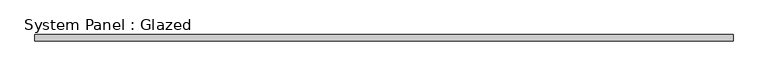
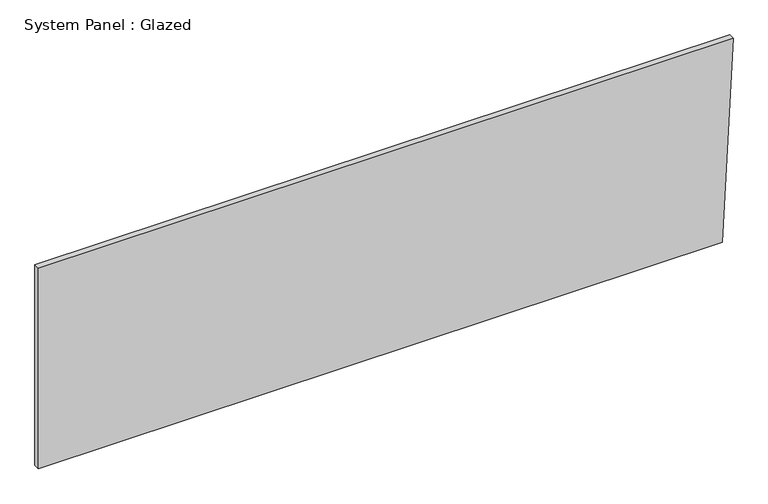
"""IFC4 building model written with IfcOpenShell, lengths in millimetres: plate geometry, System Panel : Glazed."""

from ifc_helpers import new_model, si_unit, frame, origin, place, context, project, spatial, polyline, outline, extrude, source, transform, mapped, element, save


def system_panel_glazed_eafac879(model_context):
    return source(origin(), model_context, "Body", "SweptSolid", [
        extrude(outline(polyline([(0.0, -1421.6824189), (0.0, 1376.3593837), (866.0018549, 1421.6824189), (866.0018549, -1421.6824189), (0.0, -1421.6824189)])), frame((0.0, -44.45, 0.0), z_axis=(0.0, 1.0, 0.0), x_axis=(0.0, 0.0, 1.0)), (0.0, 0.0, 1.0), 25.4),
    ])


if __name__ == "__main__":
    model = new_model("IFC4")
    model_context = context("Model", 3, world=origin())
    ifc_project = project(units=[si_unit("LENGTHUNIT", "METRE", prefix="MILLI")], contexts=[model_context])
    site = spatial("IfcSite", under=ifc_project)
    building = spatial("IfcBuilding", under=site)
    placement = place(None, origin())
    system_panel_glazed_shape = system_panel_glazed_eafac879(model_context)
    element("IfcPlate", 1, ObjectType="System Panel : Glazed", at=placement, inside=building, context=model_context, shape_type="MappedRepresentation", body=[
        mapped(system_panel_glazed_shape, transform((0.0, 0.0, 0.0), x_axis=(1.0, 0.0, 0.0), y_axis=(0.0, 1.0, 0.0), z_axis=(0.0, 0.0, 1.0))),
    ])
    save(model, "model.ifc")

# Revit data of these elements
# Type "System Panel : Glazed"
#   Construction Type Id = "GSP4R"
#   Analytic Construction = "1/8 in Pilkington single glazing"
#   Visual Light Transmittance = 0.9
#   Solar Heat Gain Coefficient = 0.86
#   Heat Transfer Coefficient (U) = 1.18115 BTU/(h·ft²·°F)
#   Define Thermal Properties by = 1
# Element 1 (IfcPlate, "System Panel : Glazed")
#   Materials on its faces: "Glass"
# Materials
#   "Glass": class "Glass", colour RGB 0 128 192, transparency 0.75, Description = "Soda Lime Glass", Cost = 0
